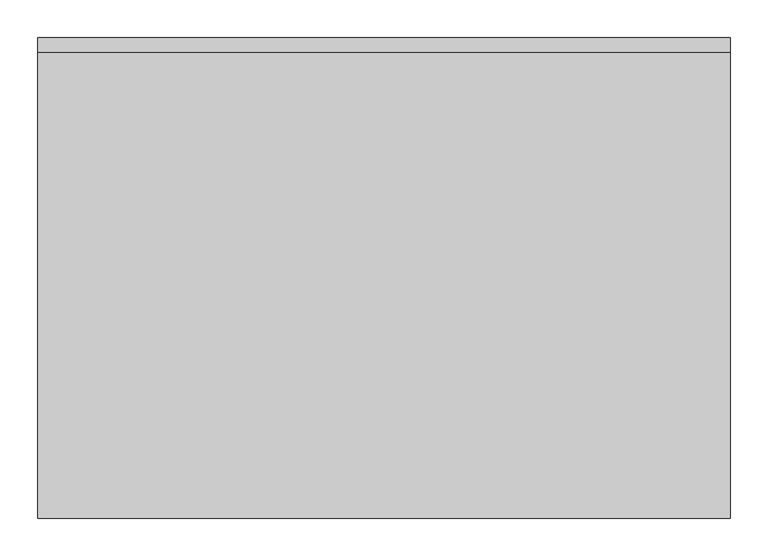
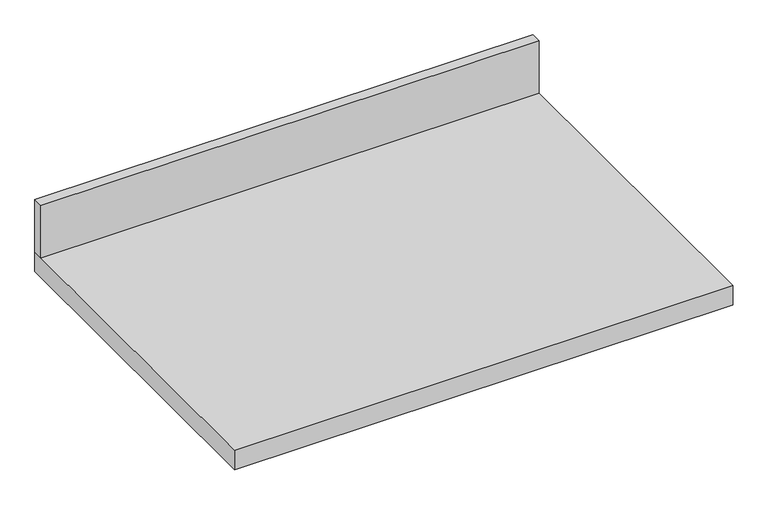
"""IFC4 building model written with IfcOpenShell, lengths in millimetres: furniture geometry, Countertop with Backsplash-NON-COLLECTUS : -."""

import ifcopenshell
import ifcopenshell.guid

model = None  # the IFC model being written
_history = None  # IfcOwnerHistory: only IFC2X3 demands one
_inside = {}  # id of a spatial element -> (the spatial element, [elements in it])
_under = {}  # id of a project, library or spatial element -> (it, [spatial elements below it])
_declared = {}  # id of a project -> (the project, [libraries it declares])
_typed = {}  # id of a type object -> (the type object, [elements of that type])
_made_of = {}  # id of a material, layer set ... -> (it, [elements and type objects made of it])


def new_model(schema):
    """Start an empty IFC model of exactly this schema.

    Asked for "IFC4X3", IfcOpenShell would pick the latest addendum, in which some entities
    have other attributes; the version numbers below select the first issue.
    IFC2X3 requires an IfcOwnerHistory on every rooted entity: one is made here for all.
    """
    global model, _history
    if schema == "IFC4X3":
        model = ifcopenshell.file(schema_version=(4, 3, 0, 0))
    else:
        model = ifcopenshell.file(schema=schema)
    _inside.clear()
    _under.clear()
    _declared.clear()
    _typed.clear()
    _made_of.clear()
    _history = None
    if model.schema == "IFC2X3":
        org = make("IfcOrganization", Name="unknown")
        user = make(
            "IfcPersonAndOrganization",
            ThePerson=make("IfcPerson", FamilyName="unknown"),
            TheOrganization=org,
        )
        app = make(
            "IfcApplication",
            ApplicationDeveloper=org,
            Version="unknown",
            ApplicationFullName="unknown",
            ApplicationIdentifier="unknown",
        )
        _history = make(
            "IfcOwnerHistory",
            OwningUser=user,
            OwningApplication=app,
            ChangeAction="ADDED",
            CreationDate=0,
        )
    return model


def make(cls, **values):
    """One entity of the class cls with the attributes given. An attribute that is None is left unset."""
    return model.create_entity(
        cls, **{name: value for name, value in values.items() if value is not None}
    )


def rooted(cls, **values):
    """An entity with a GlobalId (a new one), such as an element, a storey or a relation."""
    return make(cls, GlobalId=ifcopenshell.guid.new(), OwnerHistory=_history, **values)


def si_unit(unit_type, name, prefix=None):
    """IfcSIUnit, for example si_unit("LENGTHUNIT", "METRE", prefix="MILLI")."""
    return make("IfcSIUnit", UnitType=unit_type, Prefix=prefix, Name=name)


def assignment(units):
    """IfcUnitAssignment: the units of a project."""
    return None if units is None else make("IfcUnitAssignment", Units=units)


def point(xyz):
    """IfcCartesianPoint."""
    return None if xyz is None else make("IfcCartesianPoint", Coordinates=xyz)


def direction(xyz):
    """IfcDirection."""
    return None if xyz is None else make("IfcDirection", DirectionRatios=xyz)


def frame(location, z_axis=None, x_axis=None):
    """IfcAxis2Placement3D, a coordinate frame: its origin and axes. An axis left out is left unset."""
    return make(
        "IfcAxis2Placement3D",
        Location=point(location),
        Axis=direction(z_axis),
        RefDirection=direction(x_axis),
    )


def origin():
    """The frame at (0, 0, 0) with its axes left unset."""
    return frame((0.0, 0.0, 0.0))


def origin_with_axes():
    """The frame at (0, 0, 0) with the z axis (0, 0, 1) and the x axis (1, 0, 0) written out."""
    return frame((0.0, 0.0, 0.0), z_axis=(0.0, 0.0, 1.0), x_axis=(1.0, 0.0, 0.0))


def place(relative_to, where):
    """IfcLocalPlacement: puts the frame where relative to a parent placement (None: the world)."""
    return make(
        "IfcLocalPlacement", PlacementRelTo=relative_to, RelativePlacement=where
    )


def context(
    kind, dimensions, precision=None, world=None, true_north=None, identifier=None
):
    """IfcGeometricRepresentationContext, for example the 3D "Model" context."""
    return make(
        "IfcGeometricRepresentationContext",
        ContextIdentifier=identifier,
        ContextType=kind,
        CoordinateSpaceDimension=dimensions,
        Precision=precision,
        WorldCoordinateSystem=world,
        TrueNorth=true_north,
    )


def project(units=None, contexts=None):
    """IfcProject with its units and contexts."""
    return rooted(
        "IfcProject",
        Name="project",
        RepresentationContexts=contexts,
        UnitsInContext=assignment(units),
    )


def spatial(cls, under=None, at=None, **own):
    """A site, building, storey or space (cls), placed at a placement, below another one or the project."""
    s = rooted(cls, ObjectPlacement=at, **own)
    if under is not None:
        _under.setdefault(under.id(), (under, []))[1].append(s)
    return s


def polyline(points):
    """IfcPolyline through the points."""
    return make("IfcPolyline", Points=[point(p) for p in points])


def outline(outer, holes=None, kind="AREA"):
    """IfcArbitraryClosedProfileDef: a profile drawn as a closed curve; with holes, ...WithVoids."""
    if holes is None:
        return make("IfcArbitraryClosedProfileDef", ProfileType=kind, OuterCurve=outer)
    return make(
        "IfcArbitraryProfileDefWithVoids",
        ProfileType=kind,
        OuterCurve=outer,
        InnerCurves=holes,
    )


def extrude(swept, where, along, depth):
    """IfcExtrudedAreaSolid: the profile swept, set in the frame where, extruded along a direction by depth."""
    return make(
        "IfcExtrudedAreaSolid",
        SweptArea=swept,
        Position=where,
        ExtrudedDirection=direction(along),
        Depth=depth,
    )


def shape(context_of_items, identifier, shape_type, items):
    """IfcShapeRepresentation: the items that make up one representation, for example the "Body"."""
    return make(
        "IfcShapeRepresentation",
        ContextOfItems=context_of_items,
        RepresentationIdentifier=identifier,
        RepresentationType=shape_type,
        Items=items,
    )


def source(mapping_origin, context_of_items, identifier, shape_type, items):
    """IfcRepresentationMap: a shape defined once, which mapped items show again and again."""
    return make(
        "IfcRepresentationMap",
        MappingOrigin=mapping_origin,
        MappedRepresentation=shape(context_of_items, identifier, shape_type, items),
    )


def transform(
    local_origin,
    x_axis=None,
    y_axis=None,
    z_axis=None,
    scale=None,
    scale2=None,
    scale3=None,
    uniform=True,
):
    """IfcCartesianTransformationOperator3D, or its non-uniform kind. x_axis, y_axis, z_axis: its Axis1, 2, 3."""
    if uniform:
        return make(
            "IfcCartesianTransformationOperator3D",
            Axis1=direction(x_axis),
            Axis2=direction(y_axis),
            LocalOrigin=point(local_origin),
            Scale=scale,
            Axis3=direction(z_axis),
        )
    return make(
        "IfcCartesianTransformationOperator3DnonUniform",
        Axis1=direction(x_axis),
        Axis2=direction(y_axis),
        LocalOrigin=point(local_origin),
        Scale=scale,
        Axis3=direction(z_axis),
        Scale2=scale2,
        Scale3=scale3,
    )


def mapped(mapping_source, mapping_target):
    """IfcMappedItem: shows the shape of a source again, moved by a transform."""
    return make(
        "IfcMappedItem", MappingSource=mapping_source, MappingTarget=mapping_target
    )


def made_of(thing, what):
    """Note that an element or type object is made of a material, layer set ...; save() writes the relation."""
    if what is not None:
        _made_of.setdefault(what.id(), (what, []))[1].append(thing)
    return thing


def element(
    cls,
    number,
    at=None,
    inside=None,
    cuts=None,
    type_object=None,
    material=None,
    context=None,
    identifier="Body",
    shape_type=None,
    held_by="IfcProductDefinitionShape",
    body=None,
    shapes=None,
    **own,
):
    """One element of the class cls, such as IfcWall. Its Tag is "e" and its number.

    at: its placement. inside: the storey or other place that contains it. cuts: it is an
    opening in that element (IfcRelVoidsElement). A single representation is given by context,
    identifier, shape_type and body (its items); several are given by shapes. held_by: the class
    of the entity that holds the representations. save() writes the other relations.
    """
    e = rooted(cls, Tag="e%d" % number, ObjectPlacement=at, **own)
    if body is not None:
        shapes = [shape(context, identifier, shape_type, body)]
    if shapes is not None:
        e.Representation = make(held_by, Representations=shapes)
    if inside is not None:
        _inside.setdefault(inside.id(), (inside, []))[1].append(e)
    if cuts is not None:
        rooted(
            "IfcRelVoidsElement", RelatingBuildingElement=cuts, RelatedOpeningElement=e
        )
    if type_object is not None:
        _typed.setdefault(type_object.id(), (type_object, []))[1].append(e)
    return made_of(e, material)


def aggregate(whole, parts):
    """IfcRelAggregates: a whole, such as a stair, and the parts it consists of."""
    return rooted("IfcRelAggregates", RelatingObject=whole, RelatedObjects=parts)


def save(model, path):
    """Write the relations noted so far, then the file.

    IfcRelAggregates (storeys below a building ...), IfcRelContainedInSpatialStructure (elements
    in a storey), IfcRelDefinesByType, IfcRelAssociatesMaterial and IfcRelDeclares: one each for
    every whole, place, type object, material and project.
    """
    for whole, parts in _under.values():
        aggregate(whole, parts)
    for where, things in _inside.values():
        rooted(
            "IfcRelContainedInSpatialStructure",
            RelatedElements=things,
            RelatingStructure=where,
        )
    for kind, things in _typed.values():
        rooted("IfcRelDefinesByType", RelatedObjects=things, RelatingType=kind)
    for what, things in _made_of.values():
        rooted("IfcRelAssociatesMaterial", RelatedObjects=things, RelatingMaterial=what)
    for by, libraries in _declared.values():
        rooted("IfcRelDeclares", RelatingContext=by, RelatedDefinitions=libraries)
    model.write(path)


def furniture_850595ea(model_context):
    return source(origin(), model_context, "Body", "SweptSolid", [
        extrude(outline(polyline([(-1200.4622951, 0.0), (-286.0641239, 0.0), (-286.0641239, -19.05), (-1200.4622951, -19.05), (-1200.4622951, 0.0)])), frame((0.0, 0.0, 38.1), z_axis=(0.0, 0.0, 1.0), x_axis=(1.0, 0.0, 0.0)), (0.0, 0.0, 1.0), 101.5997206),
        extrude(outline(polyline([(-286.0641239, 0.0), (-286.0641239, -634.99873), (-1200.4622951, -634.99873), (-1200.4622951, 0.0), (-286.0641239, 0.0)])), origin_with_axes(), (0.0, 0.0, 1.0), 38.1),
    ])


if __name__ == "__main__":
    model = new_model("IFC4")
    model_context = context("Model", 3, world=origin())
    ifc_project = project(units=[si_unit("LENGTHUNIT", "METRE", prefix="MILLI")], contexts=[model_context])
    site = spatial("IfcSite", under=ifc_project)
    building = spatial("IfcBuilding", under=site)
    placement = place(None, origin())
    furniture_shape = furniture_850595ea(model_context)
    element("IfcFurniture", 1, ObjectType="Countertop with Backsplash-NON-COLLECTUS : -", at=placement, inside=building, context=model_context, shape_type="MappedRepresentation", body=[
        mapped(furniture_shape, transform((0.0, 0.0, 0.0), x_axis=(1.0, 0.0, 0.0), y_axis=(0.0, 1.0, 0.0), z_axis=(0.0, 0.0, 1.0))),
    ])
    save(model, "model.ifc")

# Revit data of these elements
# Type "Countertop with Backsplash-NON-COLLECTUS : -"
#   External ID [instance default] = ""
#   Width Reporting [instance default] = 1524 mm
#   Width [instance default] = 1524 mm
#   Height Reporting [instance default] = 139.7 mm
#   Depth Reporting [instance default] = 635 mm
#   Depth [instance default] = 635 mm
#   Height [instance default] = 139.7 mm
#   Backsplash = yes
#   Material = White
#   Default Elevation = 0
#   Assembly Code = ""
# Element 1 (IfcFurniture, "Countertop with Backsplash-NON-COLLECTUS : -")
#   Width Reporting = 914.398 mm
#   Width = 914.398 mm
#   Depth Reporting = 634.999 mm
#   Depth = 634.999 mm
#   Materials on its faces: "White"
# Materials
#   "White": class "Generic", colour RGB 255 255 255, transparency 0, Cost = 0
